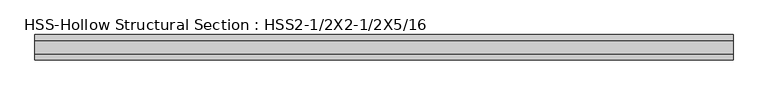
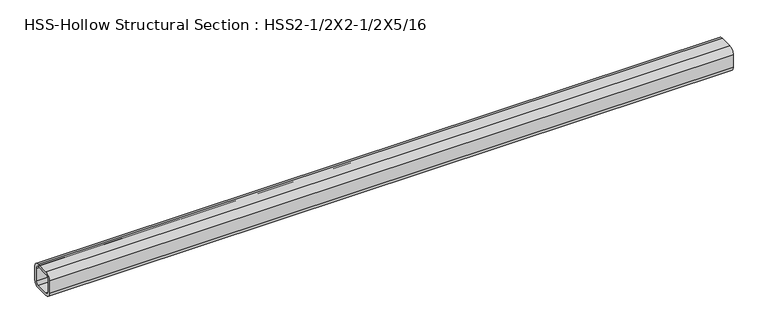
"""IFC4 building model written with IfcOpenShell, lengths in millimetres: beam geometry, HSS-Hollow Structural Section : HSS2-1/2X2-1/2X5/16."""

from ifc_helpers import new_model, si_unit, point, frame, frame_2d, origin, place, context, project, spatial, polyline, circle_curve, trimmed, segment, composite_curve, outline, extrude, source, transform, mapped, element, save


def hss_hollow_structural_section_hss2_1_2x2_1_2x5_16_7bf4390a(model_context):
    return source(origin(), model_context, "Body", "SweptSolid", [
        extrude(outline(composite_curve([segment(polyline([(31.75, 16.9672), (31.75, -16.9672)]), True, "CONTINUOUS"), segment(trimmed(circle_curve(frame_2d((16.9672, -16.9672)), 14.7828), [point((31.75, -16.9672))], [point((16.9672, -31.75))], False, "CARTESIAN"), True, "CONTINUOUS"), segment(polyline([(16.9672, -31.75), (-16.9672, -31.75)]), True, "CONTINUOUS"), segment(trimmed(circle_curve(frame_2d((-16.9672, -16.9672)), 14.7828), [point((-16.9672, -31.75))], [point((-31.75, -16.9672))], False, "CARTESIAN"), True, "CONTINUOUS"), segment(polyline([(-31.75, -16.9672), (-31.75, 16.9672)]), True, "CONTINUOUS"), segment(trimmed(circle_curve(frame_2d((-16.9672, 16.9672)), 14.7828), [point((-31.75, 16.9672))], [point((-16.9672, 31.75))], False, "CARTESIAN"), True, "CONTINUOUS"), segment(polyline([(-16.9672, 31.75), (16.9672, 31.75)]), True, "CONTINUOUS"), segment(trimmed(circle_curve(frame_2d((16.9672, 16.9672)), 14.7828), [point((16.9672, 31.75))], [point((31.75, 16.9672))], False, "CARTESIAN"), True, "CONTINUOUS")], self_intersect=False), holes=[composite_curve([segment(trimmed(circle_curve(frame_2d((-16.9672, 16.9672)), 7.3914), [point((-16.9672, 24.3586))], [point((-24.3586, 16.9672))], True, "CARTESIAN"), True, "CONTINUOUS"), segment(polyline([(-24.3586, 16.9672), (-24.3586, -16.9672)]), True, "CONTINUOUS"), segment(trimmed(circle_curve(frame_2d((-16.9672, -16.9672)), 7.3914), [point((-24.3586, -16.9672))], [point((-16.9672, -24.3586))], True, "CARTESIAN"), True, "CONTINUOUS"), segment(polyline([(-16.9672, -24.3586), (16.9672, -24.3586)]), True, "CONTINUOUS"), segment(trimmed(circle_curve(frame_2d((16.9672, -16.9672)), 7.3914), [point((16.9672, -24.3586))], [point((24.3586, -16.9672))], True, "CARTESIAN"), True, "CONTINUOUS"), segment(polyline([(24.3586, -16.9672), (24.3586, 16.9672)]), True, "CONTINUOUS"), segment(trimmed(circle_curve(frame_2d((16.9672, 16.9672)), 7.3914), [point((24.3586, 16.9672))], [point((16.9672, 24.3586))], True, "CARTESIAN"), True, "CONTINUOUS"), segment(polyline([(16.9672, 24.3586), (-16.9672, 24.3586)]), True, "CONTINUOUS")], self_intersect=False)]), frame((-906.1782689, 0.0, 0.0), z_axis=(1.0, 0.0, 0.0), x_axis=(0.0, 1.0, 0.0)), (0.0, 0.0, 1.0), 1741.6810272),
    ])


if __name__ == "__main__":
    model = new_model("IFC4")
    model_context = context("Model", 3, world=origin())
    ifc_project = project(units=[si_unit("LENGTHUNIT", "METRE", prefix="MILLI")], contexts=[model_context])
    site = spatial("IfcSite", under=ifc_project)
    building = spatial("IfcBuilding", under=site)
    placement = place(None, origin())
    hss_hollow_structural_section_hss2_1_2x2_1_2x5_16_shape = hss_hollow_structural_section_hss2_1_2x2_1_2x5_16_7bf4390a(model_context)
    element("IfcBeam", 1, ObjectType="HSS-Hollow Structural Section : HSS2-1/2X2-1/2X5/16", at=placement, inside=building, context=model_context, shape_type="MappedRepresentation", body=[
        mapped(hss_hollow_structural_section_hss2_1_2x2_1_2x5_16_shape, transform((0.0, 0.0, 0.0), x_axis=(1.0, 0.0, 0.0), y_axis=(0.0, 1.0, 0.0), z_axis=(0.0, 0.0, 1.0))),
    ])
    save(model, "model.ifc")

# Revit data of these elements
# Type "HSS-Hollow Structural Section : HSS2-1/2X2-1/2X5/16"
#   Assembly Code = "B10"
#   Shape = "Square"
#   W = 8.4
#   Ht = 0' - 2 1/2"
#   Length [instance default] = 5' - 0"
#   b = 0' - 2 1/2"
#   kr = 0' - 0.582"
#   t = 0' - 0.291"
#   A = 0.0163194 SF
#   Structural Material [instance default] = Steel ASTM A500, Grade B, Rectangular and Square
# Element 1 (IfcBeam, "HSS-Hollow Structural Section : HSS2-1/2X2-1/2X5/16")
#   Materials on its faces: "Steel ASTM A500, Grade B, Rectangular and Square"
# Materials
#   "Steel ASTM A500, Grade B, Rectangular and Square": class "Metal", colour RGB 199 199 199, transparency 0, Description = "Carbon steel", Cost = 0
